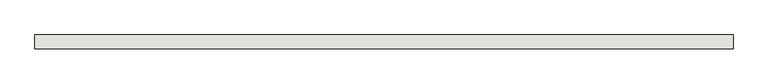
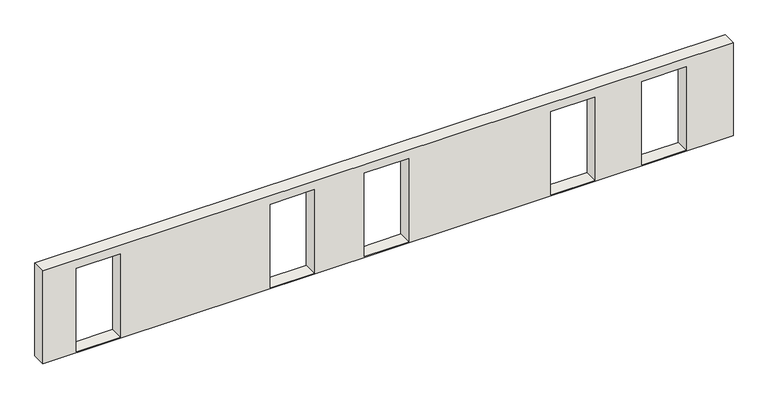
"""IFC4 building model written with IfcOpenShell, lengths in millimetres: wall geometry, 0_3d_modell."""

from ifc_helpers import new_model, si_unit, frame, origin, place, context, project, spatial, polyline, outline, extrude, source, transform, mapped, element, save


def wall_bedf632d(model_context):
    return source(origin(), model_context, "Body", "SweptSolid", [
        extrude(outline(polyline([(0.0, 0.0), (0.0, 17652.8619019), (2510.0, 17652.8619019), (2510.0, 0.0), (0.0, 0.0)]), holes=[polyline([(20.0, 12984.7954033), (2280.0, 12984.7954033), (2280.0, 14119.7954033), (20.0, 14119.7954033), (20.0, 12984.7954033)]), polyline([(20.0, 15317.8619019), (2280.0, 15317.8619019), (2280.0, 16452.8619019), (20.0, 16452.8619019), (20.0, 15317.8619019)]), polyline([(20.0, 5810.3619019), (2280.0, 5810.3619019), (2280.0, 6945.3619019), (20.0, 6945.3619019), (20.0, 5810.3619019)]), polyline([(20.0, 8224.9644869), (2280.0, 8224.9644869), (2280.0, 9359.9644869), (20.0, 9359.9644869), (20.0, 8224.9644869)]), polyline([(20.0, 850.0), (2280.0, 850.0), (2280.0, 1985.0), (20.0, 1985.0), (20.0, 850.0)])]), frame((0.0, 0.0, 0.0), z_axis=(0.0, 1.0, 0.0), x_axis=(0.0, 0.0, 1.0)), (0.0, 0.0, 1.0), 350.0),
    ])


if __name__ == "__main__":
    model = new_model("IFC4")
    model_context = context("Model", 3, world=origin())
    ifc_project = project(units=[si_unit("LENGTHUNIT", "METRE", prefix="MILLI")], contexts=[model_context])
    site = spatial("IfcSite", under=ifc_project)
    building = spatial("IfcBuilding", under=site)
    placement = place(None, origin())
    wall_shape = wall_bedf632d(model_context)
    element("IfcWall", 1, ObjectType="0_3d_modell", at=placement, inside=building, context=model_context, shape_type="MappedRepresentation", body=[
        mapped(wall_shape, transform((0.0, 0.0, 0.0), x_axis=(1.0, 0.0, 0.0), y_axis=(0.0, 1.0, 0.0), z_axis=(0.0, 0.0, 1.0))),
    ])
    save(model, "model.ifc")

# Revit data of these elements
# Element 1 (IfcWall, "0_3d_modell")
#   Materials on its faces: "holzschalung"
# Materials
#   "holzschalung": class "Unassigned", colour RGB 128 128 128, transparency 0
